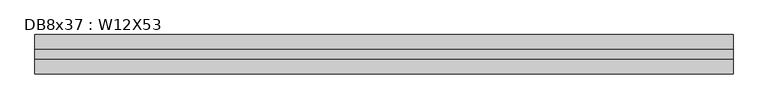
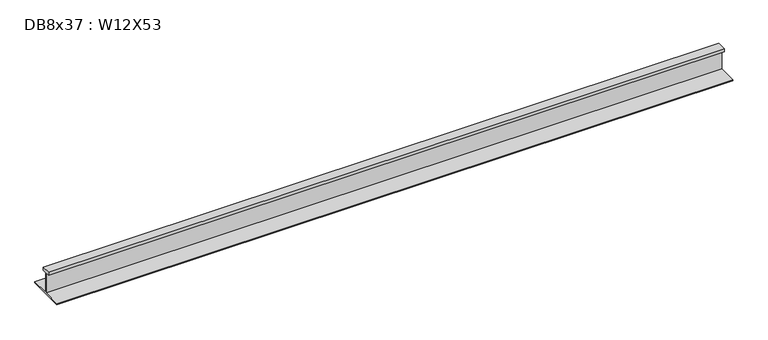
"""IFC4 building model written with IfcOpenShell, lengths in millimetres: beam geometry, DB8x37 : W12X53."""

from ifc_helpers import new_model, si_unit, frame, origin, place, context, project, spatial, polyline, outline, extrude, source, transform, mapped, element, save


def db8x37_w12x53_4241ae81(model_context):
    return source(origin(), model_context, "Body", "SweptSolid", [
        extrude(outline(polyline([(38.1, 145.415), (38.1, 120.015), (2.921, 120.015), (2.921, -48.4505), (152.4, -48.4505), (152.4, -58.1025), (-152.4, -58.1025), (-152.4, -48.4505), (-2.921, -48.4505), (-2.921, 120.015), (-38.1, 120.015), (-38.1, 145.415), (38.1, 145.415)])), frame((-2708.529, 0.0, 0.0), z_axis=(1.0, 0.0, 0.0), x_axis=(0.0, 1.0, 0.0)), (0.0, 0.0, 1.0), 5417.058),
    ])


if __name__ == "__main__":
    model = new_model("IFC4")
    model_context = context("Model", 3, world=origin())
    ifc_project = project(units=[si_unit("LENGTHUNIT", "METRE", prefix="MILLI")], contexts=[model_context])
    site = spatial("IfcSite", under=ifc_project)
    building = spatial("IfcBuilding", under=site)
    placement = place(None, origin())
    db8x37_w12x53_shape = db8x37_w12x53_4241ae81(model_context)
    element("IfcBeam", 1, ObjectType="DB8x37 : W12X53", at=placement, inside=building, context=model_context, shape_type="MappedRepresentation", body=[
        mapped(db8x37_w12x53_shape, transform((0.0, 0.0, 0.0), x_axis=(1.0, 0.0, 0.0), y_axis=(0.0, 1.0, 0.0), z_axis=(0.0, 0.0, 1.0))),
    ])
    save(model, "model.ifc")

# Revit data of these elements
# Type "DB8x37 : W12X53"
#   Assembly Code = "B10"
#   W = 53
#   Length [instance default] = 5' - 0"
#   bf = 0' - 10"
#   d = 1' - 0.1"
#   k = 0' - 1 3/8"
#   k2 = 0' - 0.8"
#   tf = 0' - 0.575"
#   tw = 0' - 0.345"
#   A = 0.108333 SF
#   Structural Material [instance default] = Steel ASTM A992
# Element 1 (IfcBeam, "DB8x37 : W12X53")
#   Materials on its faces: "Steel ASTM A992"
# Materials
#   "Steel ASTM A992": class "Metal", colour RGB 199 199 199, transparency 0, Description = "Structural steel 50ksi", Cost = 0
